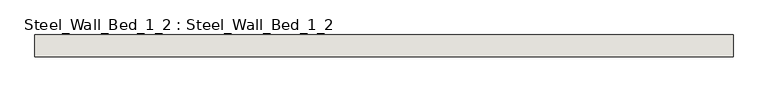
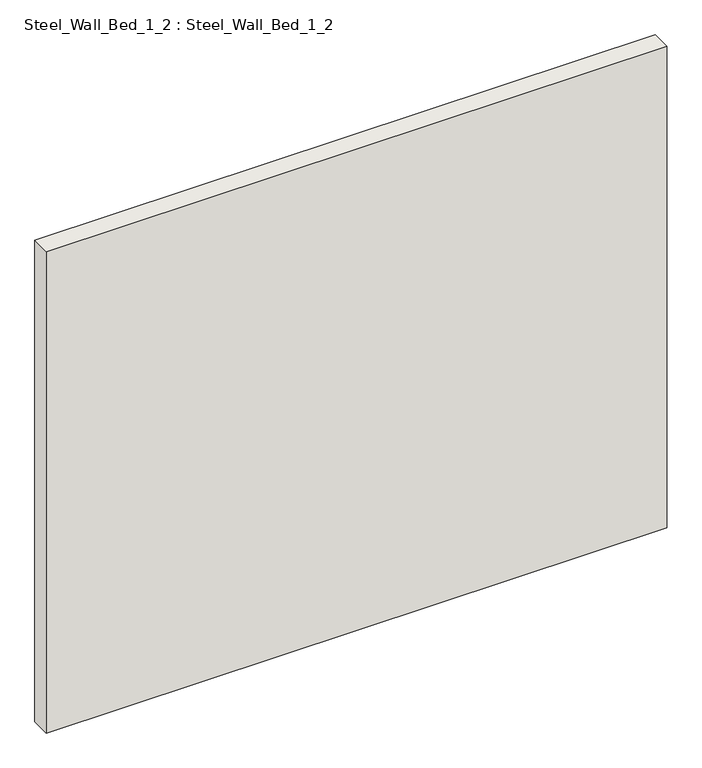
"""IFC4 building model written with IfcOpenShell, lengths in millimetres: wall geometry, Steel_Wall_Bed_1_2 : Steel_Wall_Bed_1_2."""

from ifc_helpers import new_model, si_unit, frame, origin, place, context, project, spatial, polyline, outline, extrude, source, transform, mapped, element, save


def steel_wall_bed_1_2_steel_wall_bed_1_2_5afbed24(model_context):
    return source(origin(), model_context, "Body", "SweptSolid", [
        extrude(outline(polyline([(4685.0, 4595.0), (1515.0, 4595.0), (1515.0, 4695.0), (4685.0, 4695.0), (4685.0, 4595.0)])), frame((0.0, 0.0, 250.0), z_axis=(0.0, 0.0, 1.0), x_axis=(1.0, 0.0, 0.0)), (0.0, 0.0, 1.0), 2600.0),
    ])


if __name__ == "__main__":
    model = new_model("IFC4")
    model_context = context("Model", 3, world=origin())
    ifc_project = project(units=[si_unit("LENGTHUNIT", "METRE", prefix="MILLI")], contexts=[model_context])
    site = spatial("IfcSite", under=ifc_project)
    building = spatial("IfcBuilding", under=site)
    placement = place(None, origin())
    steel_wall_bed_1_2_steel_wall_bed_1_2_shape = steel_wall_bed_1_2_steel_wall_bed_1_2_5afbed24(model_context)
    element("IfcWall", 1, ObjectType="Steel_Wall_Bed_1_2 : Steel_Wall_Bed_1_2", at=placement, inside=building, context=model_context, shape_type="MappedRepresentation", body=[
        mapped(steel_wall_bed_1_2_steel_wall_bed_1_2_shape, transform((0.0, 0.0, 0.0), x_axis=(1.0, 0.0, 0.0), y_axis=(0.0, 1.0, 0.0), z_axis=(0.0, 0.0, 1.0))),
    ])
    save(model, "model.ifc")

# Revit data of these elements
# Type "Steel_Wall_Bed_1_2 : Steel_Wall_Bed_1_2"
#   NameOverride = "Steel_Wall_Bed_1_2"
# Element 1 (IfcWall, "Steel_Wall_Bed_1_2 : Steel_Wall_Bed_1_2")
#   Materials on its faces: "IfcSurfaceStyle #33"
# Materials
#   "IfcSurfaceStyle #33": class "Unassigned", colour RGB 214 214 214, transparency 0
